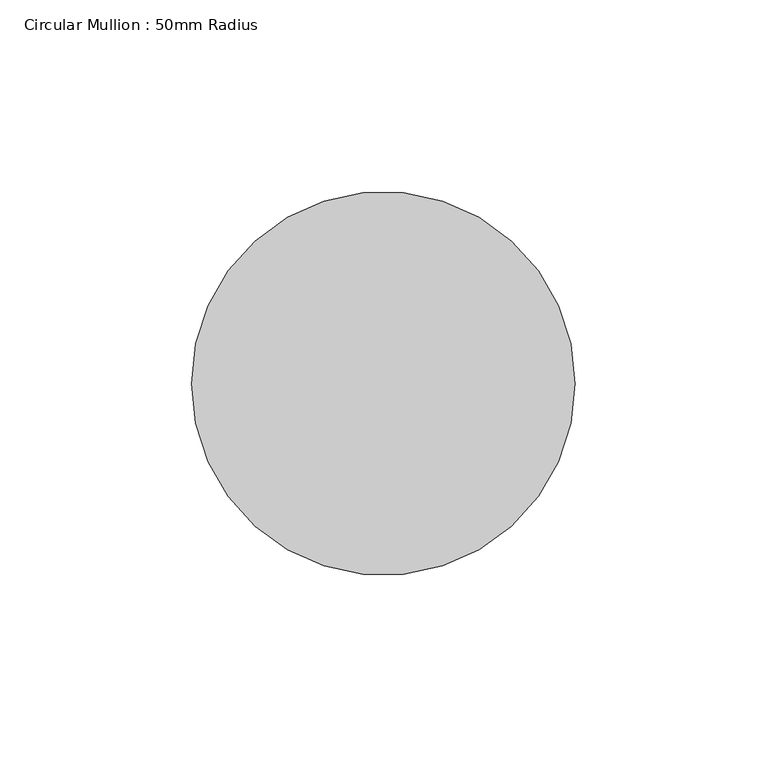
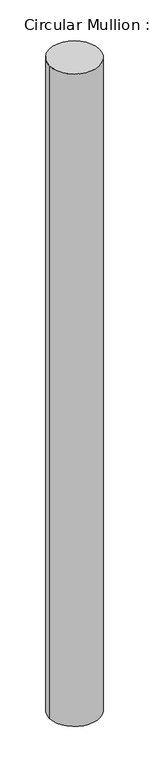
"""IFC4 building model written with IfcOpenShell, lengths in millimetres: member geometry, Circular Mullion : 50mm Radius."""

from ifc_helpers import new_model, si_unit, point, frame, origin, origin_2d, place, context, project, spatial, circle_curve, trimmed, segment, composite_curve, outline, extrude, source, transform, mapped, element, save


def circular_mullion_50mm_radius_05b3a38f(model_context):
    return source(origin(), model_context, "Body", "SweptSolid", [
        extrude(outline(composite_curve([segment(trimmed(circle_curve(origin_2d(), 50.0), [point((50.0, 0.0))], [point((-50.0, 0.0))], False, "CARTESIAN"), True, "CONTINUOUS"), segment(trimmed(circle_curve(origin_2d(), 50.0), [point((-50.0, 0.0))], [point((50.0, 0.0))], False, "CARTESIAN"), True, "CONTINUOUS")], self_intersect=False)), frame((0.0, 0.0, -1378.7368835), z_axis=(0.0, 0.0, 1.0), x_axis=(1.0, 0.0, 0.0)), (0.0, 0.0, 1.0), 1378.7368835),
    ])


if __name__ == "__main__":
    model = new_model("IFC4")
    model_context = context("Model", 3, world=origin())
    ifc_project = project(units=[si_unit("LENGTHUNIT", "METRE", prefix="MILLI")], contexts=[model_context])
    site = spatial("IfcSite", under=ifc_project)
    building = spatial("IfcBuilding", under=site)
    placement = place(None, origin())
    circular_mullion_50mm_radius_shape = circular_mullion_50mm_radius_05b3a38f(model_context)
    element("IfcMember", 1, ObjectType="Circular Mullion : 50mm Radius", at=placement, inside=building, context=model_context, shape_type="MappedRepresentation", body=[
        mapped(circular_mullion_50mm_radius_shape, transform((0.0, 0.0, 0.0), x_axis=(1.0, 0.0, 0.0), y_axis=(0.0, 1.0, 0.0), z_axis=(0.0, 0.0, 1.0))),
    ])
    save(model, "model.ifc")

# Revit data of these elements
# Type "Circular Mullion : 50mm Radius"
#   built-in parameter 1007350 = 0.164042 (stored number, unit not read)
# Element 1 (IfcMember, "Circular Mullion : 50mm Radius")
#   Materials on its faces: "Aluminium"
# Materials
#   "Aluminium": class "Metal", colour RGB 247 247 247, transparency 0, Description = "Aluminium 6061", Cost = 0
